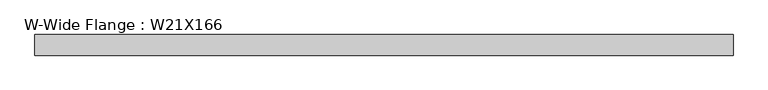
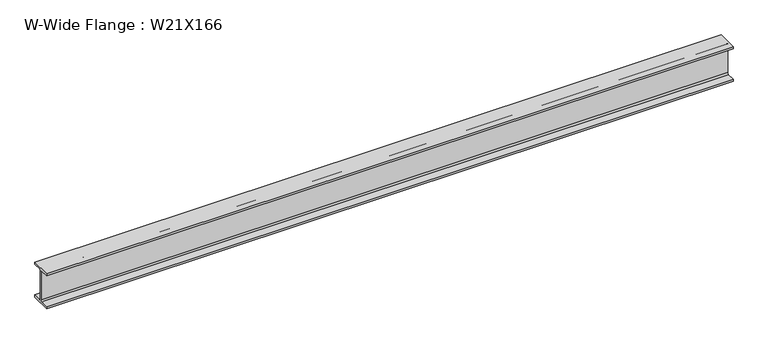
"""IFC4 building model written with IfcOpenShell, lengths in millimetres: beam geometry, W-Wide Flange : W21X166."""

from ifc_helpers import new_model, si_unit, point, frame, frame_2d, origin, place, context, project, spatial, polyline, circle_curve, trimmed, segment, composite_curve, outline, extrude, source, transform, mapped, element, save


def w_wide_flange_w21x166_c6e5425a(model_context):
    return source(origin(), model_context, "Body", "SweptSolid", [
        extrude(outline(composite_curve([segment(polyline([(157.48, -251.206), (157.48, -285.75), (-157.48, -285.75), (-157.48, -251.206), (-32.131, -251.206)]), True, "CONTINUOUS"), segment(trimmed(circle_curve(frame_2d((-32.131, -228.6)), 22.606), [point((-32.131, -251.206))], [point((-9.525, -228.6))], True, "CARTESIAN"), True, "CONTINUOUS"), segment(polyline([(-9.525, -228.6), (-9.525, 228.6)]), True, "CONTINUOUS"), segment(trimmed(circle_curve(frame_2d((-32.131, 228.6)), 22.606), [point((-9.525, 228.6))], [point((-32.131, 251.206))], True, "CARTESIAN"), True, "CONTINUOUS"), segment(polyline([(-32.131, 251.206), (-157.48, 251.206), (-157.48, 285.75), (157.48, 285.75), (157.48, 251.206), (32.131, 251.206)]), True, "CONTINUOUS"), segment(trimmed(circle_curve(frame_2d((32.131, 228.6)), 22.606), [point((32.131, 251.206))], [point((9.525, 228.6))], True, "CARTESIAN"), True, "CONTINUOUS"), segment(polyline([(9.525, 228.6), (9.525, -228.6)]), True, "CONTINUOUS"), segment(trimmed(circle_curve(frame_2d((32.131, -228.6)), 22.606), [point((9.525, -228.6))], [point((32.131, -251.206))], True, "CARTESIAN"), True, "CONTINUOUS"), segment(polyline([(32.131, -251.206), (157.48, -251.206)]), True, "CONTINUOUS")], self_intersect=False)), frame((-5453.5051023, 0.0, 0.0), z_axis=(1.0, 0.0, 0.0), x_axis=(0.0, 1.0, 0.0)), (0.0, 0.0, 1.0), 10659.8214497),
    ])


if __name__ == "__main__":
    model = new_model("IFC4")
    model_context = context("Model", 3, world=origin())
    ifc_project = project(units=[si_unit("LENGTHUNIT", "METRE", prefix="MILLI")], contexts=[model_context])
    site = spatial("IfcSite", under=ifc_project)
    building = spatial("IfcBuilding", under=site)
    placement = place(None, origin())
    w_wide_flange_w21x166_shape = w_wide_flange_w21x166_c6e5425a(model_context)
    element("IfcBeam", 1, ObjectType="W-Wide Flange : W21X166", at=placement, inside=building, context=model_context, shape_type="MappedRepresentation", body=[
        mapped(w_wide_flange_w21x166_shape, transform((0.0, 0.0, 0.0), x_axis=(1.0, 0.0, 0.0), y_axis=(0.0, 1.0, 0.0), z_axis=(0.0, 0.0, 1.0))),
    ])
    save(model, "model.ifc")

# Revit data of these elements
# Type "W-Wide Flange : W21X166"
#   Assembly Code = "B10"
#   W = 166
#   Length [instance default] = 5' - 0"
#   bf = 1' - 0.4"
#   d = 1' - 10 1/2"
#   k = 0' - 2 1/4"
#   k2 = 0' - 0.89"
#   tf = 0' - 1.36"
#   tw = 0' - 0 3/4"
#   A = 0.338889 SF
#   Structural Material [instance default] = Steel ASTM A992
# Element 1 (IfcBeam, "W-Wide Flange : W21X166")
#   Structural Material = Steel
#   Materials on its faces: "Steel"
# Materials
#   "Steel ASTM A992": class "Metal", colour RGB 199 199 199, transparency 0, Description = "Structural steel 50ksi", Cost = 0
#   "Steel": class "Metal", colour RGB 118 118 114, transparency 0, Description = "Steel, mill finish", Cost = 0
